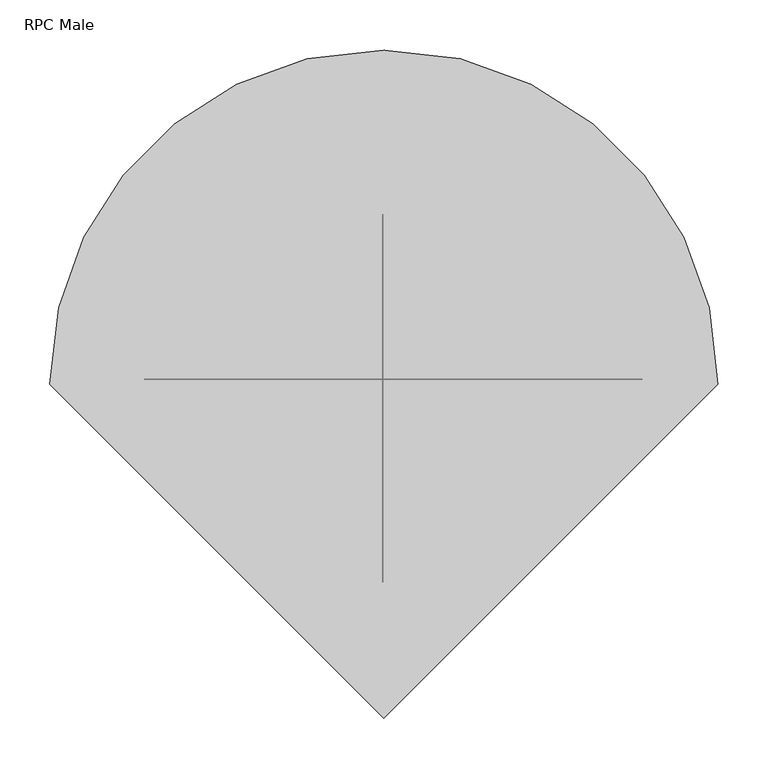
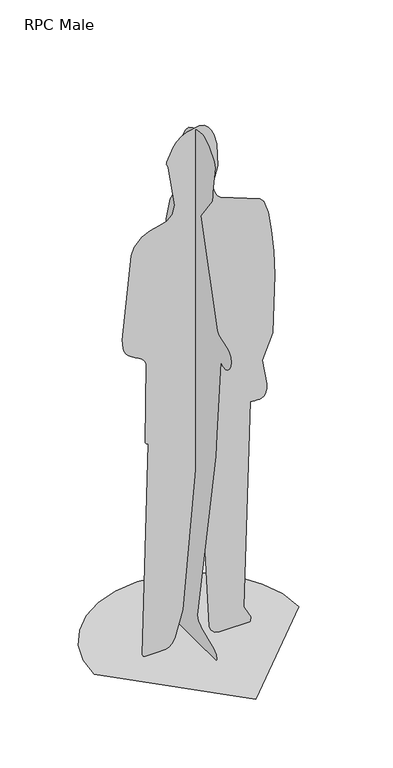
"""IFC4 building model written with IfcOpenShell, lengths in millimetres: proxy geometry, RPC Male : Dwayne."""

from ifc_helpers import new_model, si_unit, origin, place, context, project, spatial, triangles, source, transform, mapped, element, save


def rpc_male_b6464c39(model_context):
    return source(origin(), model_context, "Body", "Tessellation", [
        triangles([(-180.7519758, 4.45e-05, 5.61e-05), (-184.2427693, 8.8e-06, 2.7953145), (-186.1721755, -1.66e-05, 5.8375002), (-186.8316374, -3.35e-05, 9.127569), (-168.2846227, -8.5e-06, 733.0652109), (-173.8813015, -8.5e-06, 735.2240908), (-177.6698602, -8.1e-06, 740.93319), (-174.1985423, 8.1e-06, 1013.6682867), (-179.591309, 8.8e-06, 1024.1651751), (-188.0395216, 9.6e-06, 1032.7759867), (-198.5267085, 9.9e-06, 1040.1126028), (-210.0363257, 1.03e-05, 1046.7864687), (-221.5520472, 1.07e-05, 1053.4092476), (-232.0572199, 1.1e-05, 1060.5929661), (-240.5353907, 1.14e-05, 1068.9488514), (-245.9518842, 1.21e-05, 1078.9880642), (-249.7386988, 1.29e-05, 1091.9821838), (-252.1552483, 1.4e-05, 1106.9298906), (-253.4607645, 1.47e-05, 1122.8295742), (-224.2188539, 3.16e-05, 1405.054644), (-213.7949444, 3.31e-05, 1430.2019463), (-189.1319694, 3.46e-05, 1456.0842327), (-160.624934, 3.53e-05, 1468.8737137), (-131.9229886, 3.57e-05, 1475.6378357), (-106.6752928, 3.64e-05, 1483.4436092), (-88.5310242, 3.71e-05, 1499.3593529), (-81.1392697, 3.9e-05, 1530.4516411), (-102.942045, 4.71e-05, 1666.4696468), (-107.9472446, 4.78e-05, 1679.2650867), (-108.1474504, 4.82e-05, 1680.5741638), (-107.984815, 4.82e-05, 1682.7587688), (-107.5268306, 4.82e-05, 1685.5190655), (-106.840944, 4.86e-05, 1688.5553627), (-86.6409052, 5.11e-05, 1733.0902897), (-74.2774293, 5.19e-05, 1747.7183212), (-59.5121605, 5.26e-05, 1759.6594528), (-42.363121, 5.33e-05, 1768.7777916), (-0.9855255, 5.37e-05, 1777.9990311), (15.8808757, 5.33e-05, 1772.5528519), (29.1619555, 5.26e-05, 1761.5639877), (39.2640369, 5.19e-05, 1747.0962662), (46.5934632, 5.08e-05, 1731.2140961), (56.009163, 4.89e-05, 1695.7207684), (59.1639487, 4.41e-05, 1618.2087845), (44.4858339, 4.12e-05, 1564.7278919), (44.3096682, 4.05e-05, 1551.1862766), (46.5532813, 3.94e-05, 1537.9279289), (51.2886345, 3.86e-05, 1525.4359589), (58.5876575, 3.83e-05, 1514.1926044), (68.5223164, 3.75e-05, 1504.6808304), (198.4030241, 3.46e-05, 1454.5808361), (210.7095586, 3.38e-05, 1440.8296406), (224.9005892, 3.13e-05, 1397.8447643), (235.5369131, 2.72e-05, 1333.6069702), (242.7580384, 2.28e-05, 1256.1532677), (246.7032373, 1.77e-05, 1173.5211021), (240.2781571, 5.9e-06, 974.9290089), (206.081389, 1.1e-06, 891.6222479), (221.1961823, -4e-06, 805.6633232), (220.4650678, -5.1e-06, 788.6200321), (214.9948893, -6.3e-06, 771.8045614), (210.3552016, -6.6e-06, 765.7300776), (204.1668257, -6.6e-06, 762.0919275), (196.8959759, -7e-06, 760.3982082), (189.0090118, -7e-06, 760.1573799), (180.9721295, -7e-06, 760.8774668), (173.2515615, -6.6e-06, 762.0669291), (166.3135766, -6.6e-06, 763.2339363), (144.8011179, -4.49e-05, 59.4752896), (168.6275342, -4.74e-05, 15.3365843), (166.1985945, 4.45e-05, 5.61e-05), (66.1332089, 4.45e-05, 5.61e-05), (49.8425018, 1.03e-05, 3.9765591), (39.0246256, -1.36e-05, 14.0353), (32.5983009, -2.91e-05, 28.3297116), (-2.7441046, -9.2e-06, 720.0458748), (-54.0725034, -1.03e-05, 117.9433278), (-81.3720135, 2.13e-05, 28.0047427), (-85.5237041, 2.69e-05, 19.9172686), (-91.2433859, 3.27e-05, 12.5691172), (-99.2451413, 3.86e-05, 5.9378887), (-110.2431982, 4.45e-05, 5.61e-05), (-13.8237406, 127.6718764, 9.9621145), (-13.8237974, 127.2617633, 182.0842528), (-13.8237815, 135.2635732, 744.8695776), (-13.8237815, 136.4149928, 748.3460369), (-13.8237815, 139.3954704, 752.5736132), (-13.8237815, 143.4944026, 757.5058702), (-13.8237815, 148.0010861, 763.0962994), (-13.8237815, 152.2049901, 769.2983917), (-13.8237792, 155.3953659, 776.0656385), (-13.8237792, 156.8616281, 783.3516764), (-13.8237622, 165.9465024, 1358.6137287), (-13.8237599, 143.2743216, 1442.0927902), (-13.8237576, 71.1145501, 1552.8585583), (-13.8237576, 64.3401725, 1580.5206779), (-13.8237542, 73.5344014, 1684.7952724), (-13.8237531, 67.2131212, 1712.2161278), (-13.8237531, 55.241223, 1734.9070393), (-13.8237531, 37.9260212, 1752.7537697), (-13.8237531, 15.5748771, 1765.6426632), (-13.8237531, -11.5049084, 1773.4593372), (-13.8237531, -43.0059914, 1776.090136), (-13.8237531, -55.0860226, 1772.9164925), (-13.8237542, -79.7038559, 1756.3218658), (-13.8237554, -107.4896145, 1722.3477768), (-13.8237554, -111.5711695, 1713.01012), (-13.8237554, -112.2229284, 1702.3019073), (-13.8237588, -99.0832235, 1611.9284992), (-13.8237588, -100.6007272, 1597.8206394), (-13.8237599, -96.755177, 1579.0656796), (-13.8237622, -31.1784566, 1488.4592915), (-13.8237735, -125.7984261, 1146.7472277), (-13.8237735, -134.1993577, 1137.675107), (-13.8237747, -184.2799037, 1119.3925747), (-13.8237747, -194.4649651, 1111.9394686), (-13.8237747, -201.1343255, 1100.3801451), (-13.8237769, -203.5508567, 1084.2058416), (-13.8237769, -200.9674025, 1068.9640394), (-13.8237769, -194.2820729, 1055.8707253), (-13.8237769, -184.3928146, 1046.1415226), (-13.8237769, -172.1978105, 1040.992709), (-13.8237769, -158.595007, 1041.6399078), (-13.8237769, -144.48246, 1049.299106), (-13.8237838, -123.0429529, 785.7648285), (-13.823786, -116.906318, 707.2429499), (-13.8237928, -10.2023683, 90.6853168), (-13.823794, -17.983895, 76.1481908), (-13.8237951, -35.4714404, 63.806743), (-13.8238042, -104.5965316, 31.8661463), (-13.8238053, -119.3344402, 20.2173661), (-13.8238076, -122.9915025, 6.7192091), (-13.8238042, -122.0607091, 4.3674998), (-13.8237894, -120.3451706, 2.3141478), (-13.8237724, -119.1853577, 1.4285653), (-13.8237474, -117.8199432, 0.6534771), (-13.8237099, -116.2458387, 5.61e-05), (-13.8237077, 124.501612, 0.0), (-348.4734607, -4.7230039, 0.0001684), (-339.5987117, 72.1961519, 0.0001684), (-314.3237646, 142.8340959, 5.61e-05), (-274.6722241, 205.1669827, 5.61e-05), (-222.6681673, 257.171094, 5.61e-05), (-160.3352533, 296.8225073, 5.61e-05), (-89.6973139, 322.097527, 5.61e-05), (-12.7781649, 330.972276, 5.61e-05), (64.1409886, 322.0975634, 5.61e-05), (134.7789371, 296.8225618, 5.61e-05), (197.1118239, 257.1710577, 5.61e-05), (249.1159897, 205.1670008, 5.61e-05), (288.7673667, 142.8340595, 5.61e-05), (314.0423864, 72.1960974, 0.0001684), (322.9171354, -4.7230331, 0.0001684), (-12.7782239, -340.4182474, 0.0001684)], [[71, 70, 72], [70, 69, 72], [72, 69, 73], [73, 69, 74], [74, 69, 75], [75, 69, 76], [69, 68, 76], [1, 82, 2], [2, 82, 3], [3, 82, 4], [82, 81, 4], [81, 80, 4], [80, 79, 4], [79, 78, 4], [78, 77, 4], [4, 77, 5], [77, 76, 5], [6, 5, 7], [5, 76, 7], [7, 76, 8], [76, 68, 8], [68, 67, 8], [67, 66, 8], [66, 65, 8], [65, 64, 8], [64, 63, 8], [63, 62, 8], [62, 61, 8], [61, 60, 8], [60, 59, 8], [59, 58, 8], [58, 57, 8], [57, 56, 8], [8, 56, 9], [56, 55, 9], [9, 55, 10], [55, 54, 10], [10, 54, 11], [54, 53, 11], [11, 53, 12], [53, 52, 12], [52, 51, 12], [51, 50, 12], [12, 50, 13], [13, 50, 14], [14, 50, 15], [15, 50, 16], [16, 50, 17], [17, 50, 18], [18, 50, 19], [19, 50, 20], [20, 50, 21], [21, 50, 22], [22, 50, 23], [23, 50, 24], [24, 50, 25], [25, 50, 26], [50, 49, 26], [49, 48, 26], [26, 48, 27], [48, 47, 27], [47, 46, 27], [46, 45, 27], [45, 44, 27], [27, 44, 28], [44, 43, 28], [43, 42, 28], [28, 42, 29], [29, 42, 30], [30, 42, 31], [31, 42, 32], [32, 42, 33], [33, 42, 34], [34, 42, 35], [35, 42, 36], [36, 42, 37], [42, 41, 37], [41, 40, 37], [37, 40, 38], [38, 40, 39], [138, 137, 83], [83, 137, 84], [137, 136, 84], [136, 135, 84], [131, 130, 132], [132, 130, 133], [133, 130, 134], [134, 130, 135], [123, 122, 124], [122, 121, 124], [121, 120, 124], [120, 119, 124], [119, 118, 124], [118, 117, 124], [117, 116, 124], [116, 115, 124], [115, 114, 124], [114, 113, 124], [107, 106, 108], [106, 105, 108], [105, 104, 108], [104, 103, 108], [103, 102, 108], [102, 101, 108], [101, 100, 108], [100, 99, 108], [99, 98, 108], [98, 97, 108], [108, 97, 109], [109, 97, 110], [110, 97, 111], [97, 96, 111], [96, 95, 111], [111, 95, 112], [95, 94, 112], [94, 93, 112], [112, 93, 113], [93, 92, 113], [113, 92, 124], [124, 92, 125], [92, 91, 125], [91, 90, 125], [90, 89, 125], [89, 88, 125], [88, 87, 125], [87, 86, 125], [125, 86, 126], [86, 85, 126], [126, 85, 127], [85, 84, 127], [127, 84, 128], [84, 135, 128], [128, 135, 129], [135, 130, 129], [154, 153, 139], [153, 152, 139], [139, 152, 140], [152, 151, 140], [140, 151, 141], [141, 151, 142], [151, 150, 142], [150, 149, 142], [142, 149, 143], [143, 149, 144], [144, 149, 145], [145, 149, 146], [146, 149, 147], [147, 149, 148]], closed=False),
    ])


if __name__ == "__main__":
    model = new_model("IFC4")
    model_context = context("Model", 3, world=origin())
    ifc_project = project(units=[si_unit("LENGTHUNIT", "METRE", prefix="MILLI")], contexts=[model_context])
    site = spatial("IfcSite", under=ifc_project)
    building = spatial("IfcBuilding", under=site)
    placement = place(None, origin())
    rpc_male_shape = rpc_male_b6464c39(model_context)
    element("IfcBuildingElementProxy", 1, Name="RPC Male : Dwayne", ObjectType="RPC Male : Dwayne", at=placement, inside=building, context=model_context, shape_type="MappedRepresentation", body=[
        mapped(rpc_male_shape, transform((0.0, 0.0, 0.0), x_axis=(1.0, 0.0, 0.0), y_axis=(0.0, 1.0, 0.0), z_axis=(0.0, 0.0, 1.0))),
    ])
    save(model, "model.ifc")

# Revit data of these elements
# Type "RPC Male : Dwayne"
#   built-in parameter 1005198 = "{2, 15},{22, RPC-8-G1AE-S4G0-CKUK-A},{1, 0},{1, 0},{2, 15},{1, 8},{5, Color},{1, 0},{1, 0},{3, 0.8},{3, 0.8},{3, 0.8},{1, 8},{7, BBoxMin},{1, 0},{1, 0},{1, 0},{1, 0},{1, 0},{1, 8},{7, BBoxMax},{1, 0},{1, 0},{1, 0},{1, 0},{1, 0},{2, 11},{9, RPCTypeId},{1, 0},{1, 0},{22, RPC-8-G1AE-S4G0-CKUK-A},{1, 6},{14, RPCPlantHeight},{1, 0},{1, 0},{7, 5.83333},{2, 11},{7, keyword},{1, 0},{1, 0},{45, :RPCs:People [Business-Hispanic]:Geometry:RPC},{2, 11},{8, category},{1, 0},{1, 0},{26, People [Business-Hispanic]},{2, 11},{12, LocalizedUID},{1, 0},{1, 0},{6, Dwayne},{2, 14},{6, Height},{1, 0},{1, 0},{7, 5.83333},{1, 2},{16, Cast Reflections},{1, 0},{1, 0},{1, 0},{1, 2},{6, Jitter},{1, 0},{1, 0},{1, 1},{1, 2},{9, Billboard},{1, 0},{1, 0},{1, 0},{1, 2},{12, Cast Shadows},{1, 0},{1, 0},{1, 1},{1, 2},{20, Apply Filter Effects},{1, 0},{1, 0},{1, 0},{2, 11},{28, Apply Filter Effects-Text-FC},{1, 0},{1, 0},{4, None},{21, assetlibrary_base.fbx},{1, 5},"
#   built-in parameter 1005195 = "RPC-8-G1AE-S4G0-CKUK-A"
#   Height = 0
